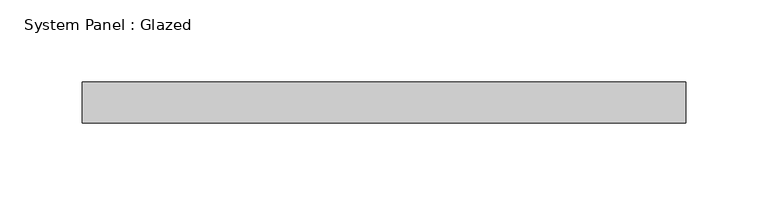
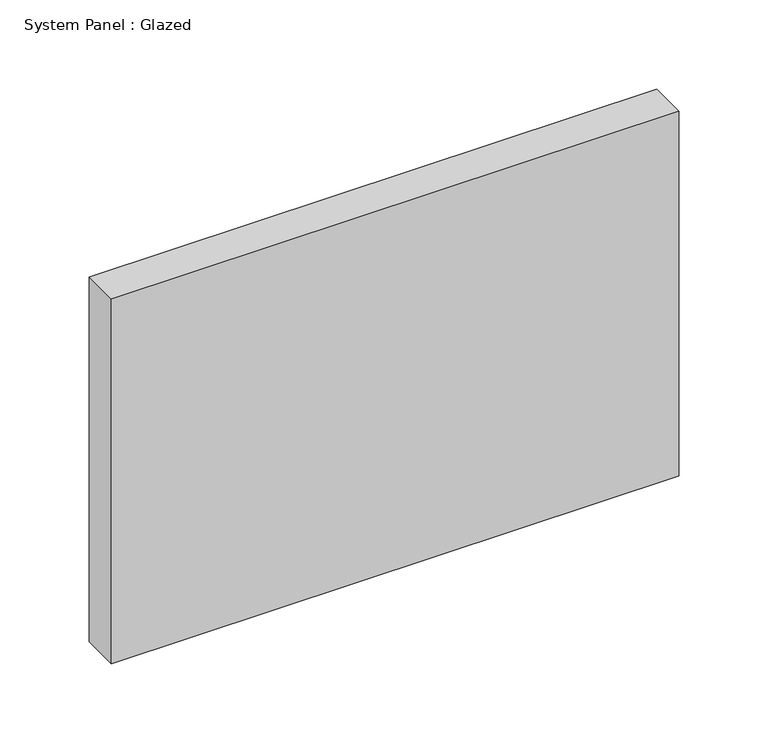
"""IFC4 building model written with IfcOpenShell, lengths in millimetres: plate geometry, System Panel : Glazed."""

from ifc_helpers import new_model, si_unit, origin, origin_with_axes, place, context, project, spatial, polyline, outline, extrude, source, transform, mapped, element, save


def system_panel_glazed_e55412e3(model_context):
    return source(origin(), model_context, "Body", "SweptSolid", [
        extrude(outline(polyline([(183.8383838, 24.5), (-183.8383838, 24.5), (-183.8383838, 49.5), (183.8383838, 49.5), (183.8383838, 24.5)])), origin_with_axes(), (0.0, 0.0, 1.0), 250.0),
    ])


if __name__ == "__main__":
    model = new_model("IFC4")
    model_context = context("Model", 3, world=origin())
    ifc_project = project(units=[si_unit("LENGTHUNIT", "METRE", prefix="MILLI")], contexts=[model_context])
    site = spatial("IfcSite", under=ifc_project)
    building = spatial("IfcBuilding", under=site)
    placement = place(None, origin())
    system_panel_glazed_shape = system_panel_glazed_e55412e3(model_context)
    element("IfcPlate", 1, ObjectType="System Panel : Glazed", at=placement, inside=building, context=model_context, shape_type="MappedRepresentation", body=[
        mapped(system_panel_glazed_shape, transform((0.0, 0.0, 0.0), x_axis=(1.0, 0.0, 0.0), y_axis=(0.0, 1.0, 0.0), z_axis=(0.0, 0.0, 1.0))),
    ])
    save(model, "model.ifc")

# Revit data of these elements
# Element 1 (IfcPlate, "System Panel : Glazed")
#   Materials on its faces: "Glass"
# Materials
#   "Glass": class "Glass", colour RGB 218 227 224, transparency 0.85, Description = "Soda Lime Glass", Cost = 0
